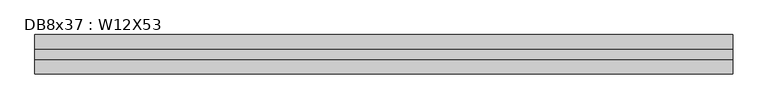
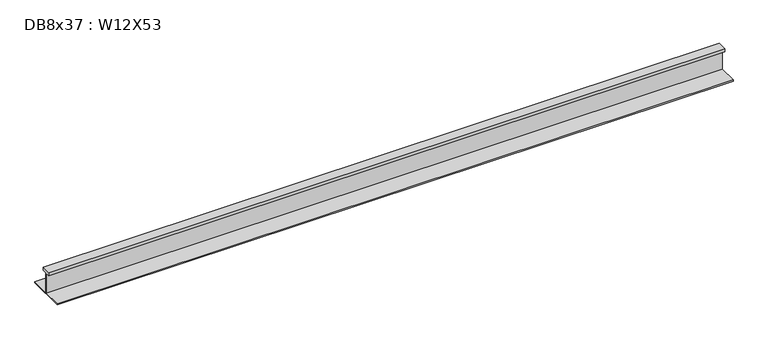
"""IFC4 building model written with IfcOpenShell, lengths in millimetres: beam geometry, DB8x37 : W12X53."""

from ifc_helpers import new_model, si_unit, frame, origin, place, context, project, spatial, polyline, outline, extrude, source, transform, mapped, element, save


def db8x37_w12x53_813fb5bc(model_context):
    return source(origin(), model_context, "Body", "SweptSolid", [
        extrude(outline(polyline([(38.1, 145.415), (38.1, 120.015), (2.921, 120.015), (2.921, -48.4505), (152.4, -48.4505), (152.4, -58.1025), (-152.4, -58.1025), (-152.4, -48.4505), (-2.921, -48.4505), (-2.921, 120.015), (-38.1, 120.015), (-38.1, 145.415), (38.1, 145.415)])), frame((-2692.4, 0.0, 0.0), z_axis=(1.0, 0.0, 0.0), x_axis=(0.0, 1.0, 0.0)), (0.0, 0.0, 1.0), 5384.8),
    ])


if __name__ == "__main__":
    model = new_model("IFC4")
    model_context = context("Model", 3, world=origin())
    ifc_project = project(units=[si_unit("LENGTHUNIT", "METRE", prefix="MILLI")], contexts=[model_context])
    site = spatial("IfcSite", under=ifc_project)
    building = spatial("IfcBuilding", under=site)
    placement = place(None, origin())
    db8x37_w12x53_shape = db8x37_w12x53_813fb5bc(model_context)
    element("IfcBeam", 1, ObjectType="DB8x37 : W12X53", at=placement, inside=building, context=model_context, shape_type="MappedRepresentation", body=[
        mapped(db8x37_w12x53_shape, transform((0.0, 0.0, 0.0), x_axis=(1.0, 0.0, 0.0), y_axis=(0.0, 1.0, 0.0), z_axis=(0.0, 0.0, 1.0))),
    ])
    save(model, "model.ifc")

# Revit data of these elements
# Type "DB8x37 : W12X53"
#   Assembly Code = "B10"
#   W = 53
#   Length [instance default] = 5' - 0"
#   bf = 0' - 10"
#   d = 1' - 0.1"
#   k = 0' - 1 3/8"
#   k2 = 0' - 0.8"
#   tf = 0' - 0.575"
#   tw = 0' - 0.345"
#   A = 0.108333 SF
#   Structural Material [instance default] = Steel ASTM A992
# Element 1 (IfcBeam, "DB8x37 : W12X53")
#   Materials on its faces: "Steel ASTM A992"
# Materials
#   "Steel ASTM A992": class "Metal", colour RGB 199 199 199, transparency 0, Description = "Structural steel 50ksi", Cost = 0
